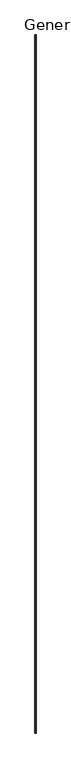
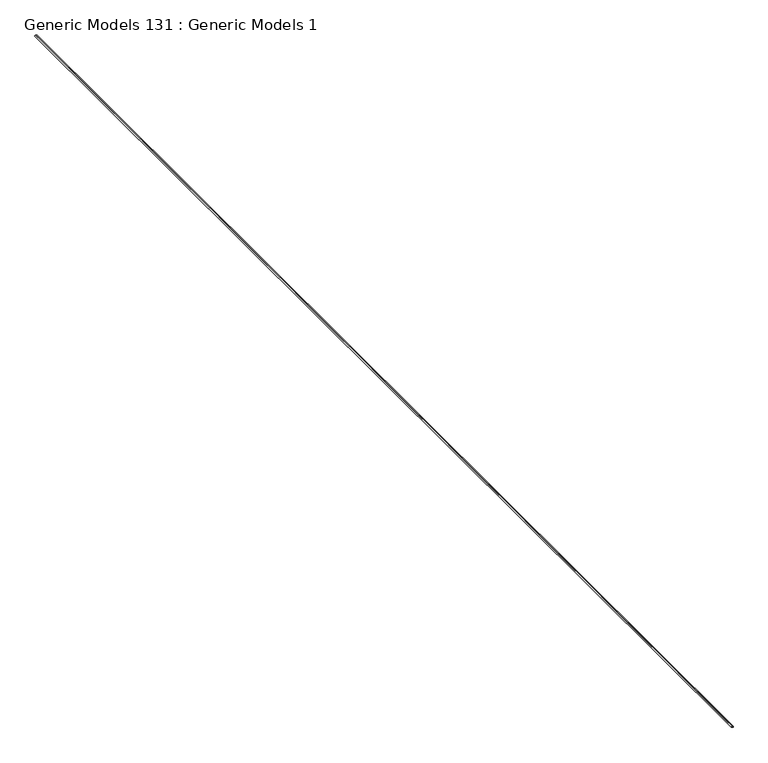
"""IFC4 building model written with IfcOpenShell, lengths in millimetres: proxy geometry, Generic Models 131 : Generic Models 1."""

import ifcopenshell
import ifcopenshell.guid

model = None  # the IFC model being written
_history = None  # IfcOwnerHistory: only IFC2X3 demands one
_inside = {}  # id of a spatial element -> (the spatial element, [elements in it])
_under = {}  # id of a project, library or spatial element -> (it, [spatial elements below it])
_declared = {}  # id of a project -> (the project, [libraries it declares])
_typed = {}  # id of a type object -> (the type object, [elements of that type])
_made_of = {}  # id of a material, layer set ... -> (it, [elements and type objects made of it])


def new_model(schema):
    """Start an empty IFC model of exactly this schema.

    Asked for "IFC4X3", IfcOpenShell would pick the latest addendum, in which some entities
    have other attributes; the version numbers below select the first issue.
    IFC2X3 requires an IfcOwnerHistory on every rooted entity: one is made here for all.
    """
    global model, _history
    if schema == "IFC4X3":
        model = ifcopenshell.file(schema_version=(4, 3, 0, 0))
    else:
        model = ifcopenshell.file(schema=schema)
    _inside.clear()
    _under.clear()
    _declared.clear()
    _typed.clear()
    _made_of.clear()
    _history = None
    if model.schema == "IFC2X3":
        org = make("IfcOrganization", Name="unknown")
        user = make(
            "IfcPersonAndOrganization",
            ThePerson=make("IfcPerson", FamilyName="unknown"),
            TheOrganization=org,
        )
        app = make(
            "IfcApplication",
            ApplicationDeveloper=org,
            Version="unknown",
            ApplicationFullName="unknown",
            ApplicationIdentifier="unknown",
        )
        _history = make(
            "IfcOwnerHistory",
            OwningUser=user,
            OwningApplication=app,
            ChangeAction="ADDED",
            CreationDate=0,
        )
    return model


def make(cls, **values):
    """One entity of the class cls with the attributes given. An attribute that is None is left unset."""
    return model.create_entity(
        cls, **{name: value for name, value in values.items() if value is not None}
    )


def rooted(cls, **values):
    """An entity with a GlobalId (a new one), such as an element, a storey or a relation."""
    return make(cls, GlobalId=ifcopenshell.guid.new(), OwnerHistory=_history, **values)


def si_unit(unit_type, name, prefix=None):
    """IfcSIUnit, for example si_unit("LENGTHUNIT", "METRE", prefix="MILLI")."""
    return make("IfcSIUnit", UnitType=unit_type, Prefix=prefix, Name=name)


def assignment(units):
    """IfcUnitAssignment: the units of a project."""
    return None if units is None else make("IfcUnitAssignment", Units=units)


def point(xyz):
    """IfcCartesianPoint."""
    return None if xyz is None else make("IfcCartesianPoint", Coordinates=xyz)


def direction(xyz):
    """IfcDirection."""
    return None if xyz is None else make("IfcDirection", DirectionRatios=xyz)


def frame(location, z_axis=None, x_axis=None):
    """IfcAxis2Placement3D, a coordinate frame: its origin and axes. An axis left out is left unset."""
    return make(
        "IfcAxis2Placement3D",
        Location=point(location),
        Axis=direction(z_axis),
        RefDirection=direction(x_axis),
    )


def origin():
    """The frame at (0, 0, 0) with its axes left unset."""
    return frame((0.0, 0.0, 0.0))


def place(relative_to, where):
    """IfcLocalPlacement: puts the frame where relative to a parent placement (None: the world)."""
    return make(
        "IfcLocalPlacement", PlacementRelTo=relative_to, RelativePlacement=where
    )


def context(
    kind, dimensions, precision=None, world=None, true_north=None, identifier=None
):
    """IfcGeometricRepresentationContext, for example the 3D "Model" context."""
    return make(
        "IfcGeometricRepresentationContext",
        ContextIdentifier=identifier,
        ContextType=kind,
        CoordinateSpaceDimension=dimensions,
        Precision=precision,
        WorldCoordinateSystem=world,
        TrueNorth=true_north,
    )


def project(units=None, contexts=None):
    """IfcProject with its units and contexts."""
    return rooted(
        "IfcProject",
        Name="project",
        RepresentationContexts=contexts,
        UnitsInContext=assignment(units),
    )


def spatial(cls, under=None, at=None, **own):
    """A site, building, storey or space (cls), placed at a placement, below another one or the project."""
    s = rooted(cls, ObjectPlacement=at, **own)
    if under is not None:
        _under.setdefault(under.id(), (under, []))[1].append(s)
    return s


def polyline(points):
    """IfcPolyline through the points."""
    return make("IfcPolyline", Points=[point(p) for p in points])


def circle_curve(where, radius):
    """IfcCircle in the frame where."""
    return make("IfcCircle", Position=where, Radius=radius)


def ellipse_curve(where, semi_axis1, semi_axis2):
    """IfcEllipse in the frame where."""
    return make(
        "IfcEllipse", Position=where, SemiAxis1=semi_axis1, SemiAxis2=semi_axis2
    )


def trimmed(basis, trim1, trim2, sense, master):
    """IfcTrimmedCurve: the piece of a basis curve between two trims."""
    return make(
        "IfcTrimmedCurve",
        BasisCurve=basis,
        Trim1=trim1,
        Trim2=trim2,
        SenseAgreement=sense,
        MasterRepresentation=master,
    )


def shape(context_of_items, identifier, shape_type, items):
    """IfcShapeRepresentation: the items that make up one representation, for example the "Body"."""
    return make(
        "IfcShapeRepresentation",
        ContextOfItems=context_of_items,
        RepresentationIdentifier=identifier,
        RepresentationType=shape_type,
        Items=items,
    )


def source(mapping_origin, context_of_items, identifier, shape_type, items):
    """IfcRepresentationMap: a shape defined once, which mapped items show again and again."""
    return make(
        "IfcRepresentationMap",
        MappingOrigin=mapping_origin,
        MappedRepresentation=shape(context_of_items, identifier, shape_type, items),
    )


def transform(
    local_origin,
    x_axis=None,
    y_axis=None,
    z_axis=None,
    scale=None,
    scale2=None,
    scale3=None,
    uniform=True,
):
    """IfcCartesianTransformationOperator3D, or its non-uniform kind. x_axis, y_axis, z_axis: its Axis1, 2, 3."""
    if uniform:
        return make(
            "IfcCartesianTransformationOperator3D",
            Axis1=direction(x_axis),
            Axis2=direction(y_axis),
            LocalOrigin=point(local_origin),
            Scale=scale,
            Axis3=direction(z_axis),
        )
    return make(
        "IfcCartesianTransformationOperator3DnonUniform",
        Axis1=direction(x_axis),
        Axis2=direction(y_axis),
        LocalOrigin=point(local_origin),
        Scale=scale,
        Axis3=direction(z_axis),
        Scale2=scale2,
        Scale3=scale3,
    )


def mapped(mapping_source, mapping_target):
    """IfcMappedItem: shows the shape of a source again, moved by a transform."""
    return make(
        "IfcMappedItem", MappingSource=mapping_source, MappingTarget=mapping_target
    )


def made_of(thing, what):
    """Note that an element or type object is made of a material, layer set ...; save() writes the relation."""
    if what is not None:
        _made_of.setdefault(what.id(), (what, []))[1].append(thing)
    return thing


def element(
    cls,
    number,
    at=None,
    inside=None,
    cuts=None,
    type_object=None,
    material=None,
    context=None,
    identifier="Body",
    shape_type=None,
    held_by="IfcProductDefinitionShape",
    body=None,
    shapes=None,
    **own,
):
    """One element of the class cls, such as IfcWall. Its Tag is "e" and its number.

    at: its placement. inside: the storey or other place that contains it. cuts: it is an
    opening in that element (IfcRelVoidsElement). A single representation is given by context,
    identifier, shape_type and body (its items); several are given by shapes. held_by: the class
    of the entity that holds the representations. save() writes the other relations.
    """
    e = rooted(cls, Tag="e%d" % number, ObjectPlacement=at, **own)
    if body is not None:
        shapes = [shape(context, identifier, shape_type, body)]
    if shapes is not None:
        e.Representation = make(held_by, Representations=shapes)
    if inside is not None:
        _inside.setdefault(inside.id(), (inside, []))[1].append(e)
    if cuts is not None:
        rooted(
            "IfcRelVoidsElement", RelatingBuildingElement=cuts, RelatedOpeningElement=e
        )
    if type_object is not None:
        _typed.setdefault(type_object.id(), (type_object, []))[1].append(e)
    return made_of(e, material)


def aggregate(whole, parts):
    """IfcRelAggregates: a whole, such as a stair, and the parts it consists of."""
    return rooted("IfcRelAggregates", RelatingObject=whole, RelatedObjects=parts)


def save(model, path):
    """Write the relations noted so far, then the file.

    IfcRelAggregates (storeys below a building ...), IfcRelContainedInSpatialStructure (elements
    in a storey), IfcRelDefinesByType, IfcRelAssociatesMaterial and IfcRelDeclares: one each for
    every whole, place, type object, material and project.
    """
    for whole, parts in _under.values():
        aggregate(whole, parts)
    for where, things in _inside.values():
        rooted(
            "IfcRelContainedInSpatialStructure",
            RelatedElements=things,
            RelatingStructure=where,
        )
    for kind, things in _typed.values():
        rooted("IfcRelDefinesByType", RelatedObjects=things, RelatingType=kind)
    for what, things in _made_of.values():
        rooted("IfcRelAssociatesMaterial", RelatedObjects=things, RelatingMaterial=what)
    for by, libraries in _declared.values():
        rooted("IfcRelDeclares", RelatingContext=by, RelatedDefinitions=libraries)
    model.write(path)


def plane_surface(at):
    """IfcPlane: the flat surface through the origin of the frame at, square to its z axis."""
    return make("IfcPlane", Position=at)


def cylinder_surface(at, radius):
    """IfcCylindricalSurface: all points at the distance radius from the z axis of the frame at."""
    return make("IfcCylindricalSurface", Position=at, Radius=radius)


def revolved_surface(curve, axis_point, axis_direction):
    """IfcSurfaceOfRevolution: the curve turned about the line through axis_point along axis_direction."""
    return make(
        "IfcSurfaceOfRevolution",
        SweptCurve=make("IfcArbitraryOpenProfileDef", ProfileType="CURVE", Curve=curve),
        AxisPosition=make("IfcAxis1Placement", Location=point(axis_point), Axis=direction(axis_direction)),
    )


def extruded_surface(curve, direction_of_extrusion, depth):
    """IfcSurfaceOfLinearExtrusion: the curve pushed along a direction by depth."""
    return make(
        "IfcSurfaceOfLinearExtrusion",
        SweptCurve=make("IfcArbitraryOpenProfileDef", ProfileType="CURVE", Curve=curve),
        ExtrudedDirection=direction(direction_of_extrusion),
        Depth=depth,
    )


def advanced_brep(points, edges, surfaces, faces):
    """IfcAdvancedBrep: a solid bounded by faces that lie on surfaces and meet in shared edges.

    An edge is (start, end): straight between two places in points (the first is 0);
    or (start, end, curve); or (start, end, curve, False) where it runs against its curve.
    A face is (place in surfaces, loops), or (place, loops, False) where it looks against
    its surface's normal. A loop lists edges by number (the first is 1), with a minus sign
    where the edge is run from its end to its start. The first loop is the outer one.
    """
    corners = [point(p) for p in points]
    vertices = [make("IfcVertexPoint", VertexGeometry=c) for c in corners]
    made = []
    for start, end, *more in edges:
        made.append(
            make(
                "IfcEdgeCurve",
                EdgeStart=vertices[start],
                EdgeEnd=vertices[end],
                EdgeGeometry=more[0] if more else make("IfcPolyline", Points=[corners[start], corners[end]]),
                SameSense=more[1] if len(more) > 1 else True,
            )
        )
    hull = []
    for where, loops, *sense in faces:
        bounds = []
        for j, loop in enumerate(loops):
            ring = [make("IfcOrientedEdge", EdgeElement=made[abs(k) - 1], Orientation=k > 0) for k in loop]
            bounds.append(
                make(
                    "IfcFaceOuterBound" if j == 0 else "IfcFaceBound",
                    Bound=make("IfcEdgeLoop", EdgeList=ring),
                    Orientation=True,
                )
            )
        hull.append(make("IfcAdvancedFace", Bounds=bounds, FaceSurface=surfaces[where], SameSense=sense[0] if sense else True))
    return make("IfcAdvancedBrep", Outer=make("IfcClosedShell", CfsFaces=hull))


def generic_models_131_generic_models_1_40819db8(model_context):
    return source(origin(), model_context, "Body", "AdvancedBrep", [
        advanced_brep(
        [(5019.461606, -1504.2676118, 129170.1348752), (5016.286606, -1504.2676118, 129170.1348752), (5015.3348467, -1504.2676118, 129168.8642166), (5015.3348467, -1504.2676118, 129165.0555337), (5016.286606, -1504.2676118, 129163.7848752), (5019.461606, -1504.2676118, 129163.7848752), (5019.461606, 6382.4323882, 129170.1348752), (5019.461606, 6382.4323882, 129163.7848752), (5016.286606, 6382.4323882, 129163.7848752), (5015.3348467, 6382.4323882, 129165.0555337), (5015.3348467, 6382.4323882, 129168.8642166), (5016.286606, 6382.4323882, 129170.1348752)],
        [
            (0, 1),
            (1, 2, circle_curve(frame((5019.2013465, -1504.2676118, 129166.9598752), z_axis=(0.0, -1.0, 0.0), x_axis=(0.0, 0.0, 1.0)), 4.3100275)),
            (2, 3, ellipse_curve(frame((5011.524106, -1504.2676118, 129166.9598752), z_axis=(0.0, -1.0, 0.0), x_axis=(1.0, 0.0, 0.0)), 4.7625, 3.175)),
            (3, 4, circle_curve(frame((5019.2013465, -1504.2676118, 129166.9598752), z_axis=(0.0, -1.0, 0.0), x_axis=(0.0, 0.0, 1.0)), 4.3100275)),
            (4, 5),
            (5, 0, circle_curve(frame((5022.3763465, -1504.2676118, 129166.9598752), z_axis=(0.0, 1.0, 0.0), x_axis=(0.0, 0.0, 1.0)), 4.3100275)),
            (6, 7, circle_curve(frame((5022.3763465, 6382.4323882, 129166.9598752), z_axis=(0.0, -1.0, 0.0), x_axis=(0.0, 0.0, 1.0)), 4.3100275)),
            (7, 8),
            (8, 9, circle_curve(frame((5019.2013465, 6382.4323882, 129166.9598752), z_axis=(0.0, 1.0, 0.0), x_axis=(0.0, 0.0, 1.0)), 4.3100275)),
            (9, 10, ellipse_curve(frame((5011.524106, 6382.4323882, 129166.9598752), z_axis=(0.0, 1.0, 0.0), x_axis=(1.0, 0.0, 0.0)), 4.7625, 3.175)),
            (10, 11, circle_curve(frame((5019.2013465, 6382.4323882, 129166.9598752), z_axis=(0.0, 1.0, 0.0), x_axis=(0.0, 0.0, 1.0)), 4.3100275)),
            (11, 6),
            (2, 10),
            (9, 3),
            (0, 6),
            (11, 1),
            (8, 4),
            (7, 5),
        ],
        [
            plane_surface(frame((5019.461606, -1504.2676118, 129163.7848752), z_axis=(0.0, -1.0, 0.0), x_axis=(1.0, 0.0, 0.0))),
            plane_surface(frame((5019.461606, 6382.4323882, 129163.7848752), z_axis=(0.0, 1.0, 0.0), x_axis=(1.0, 0.0, 0.0))),
            extruded_surface(trimmed(ellipse_curve(frame((5011.524106, 6382.4323882, 129166.9598752), z_axis=(0.0, -1.0, 0.0), x_axis=(1.0, 0.0, 0.0)), 4.7625, 3.175), [point((5015.3348467, 6382.4323882, 129168.8642166))], [point((5015.3348467, 6382.4323882, 129165.0555337))], True, "CARTESIAN"), (0.0, -7886.7, 0.0), 7886.7),
            plane_surface(frame((5019.461606, -1504.2676118, 129170.1348752), z_axis=(0.0, 0.0, 1.0), x_axis=(0.0, 1.0, 0.0))),
            cylinder_surface(frame((5019.2013465, -1504.2676118, 129166.9598752), z_axis=(0.0, -1.0, 0.0), x_axis=(0.0, 0.0, 1.0)), 4.3100275),
            plane_surface(frame((5016.286606, -1504.2676118, 129163.7848752), z_axis=(0.0, 0.0, -1.0), x_axis=(0.0, 1.0, 0.0))),
            revolved_surface(polyline([(5022.3763465, 6382.4323882, 129171.2699027), (5022.3763465, -1504.2676118, 129171.2699027)]), (5022.3763465, -1504.2676118, 129166.9598752), (0.0, 1.0, 0.0)),
        ],
        [
            (0, [[1, 2, 3, 4, 5, 6]]),
            (1, [[7, 8, 9, 10, 11, 12]]),
            (2, [[-3, 13, -10, 14]]),
            (3, [[-1, 15, -12, 16]]),
            (4, [[-4, -14, -9, 17]]),
            (5, [[-5, -17, -8, 18]]),
            (6, [[-6, -18, -7, -15]]),
            (4, [[-2, -16, -11, -13]]),
        ],
    ),
    ])


if __name__ == "__main__":
    model = new_model("IFC4")
    model_context = context("Model", 3, world=origin())
    ifc_project = project(units=[si_unit("LENGTHUNIT", "METRE", prefix="MILLI")], contexts=[model_context])
    site = spatial("IfcSite", under=ifc_project)
    building = spatial("IfcBuilding", under=site)
    placement = place(None, origin())
    generic_models_131_generic_models_1_shape = generic_models_131_generic_models_1_40819db8(model_context)
    element("IfcBuildingElementProxy", 1, Name="Generic Models 131 : Generic Models 1", ObjectType="Generic Models 131 : Generic Models 1", at=placement, inside=building, context=model_context, shape_type="MappedRepresentation", body=[
        mapped(generic_models_131_generic_models_1_shape, transform((0.0, 0.0, 0.0), x_axis=(1.0, 0.0, 0.0), y_axis=(0.0, 1.0, 0.0), z_axis=(0.0, 0.0, 1.0))),
    ])
    save(model, "model.ifc")

# Revit data of these elements
# Element 1 (IfcBuildingElementProxy, "Generic Models 131 : Generic Models 1")
#   Materials on its faces: "_SEALANT AND BACKROD, IF NEC."
# Materials
#   "_SEALANT AND BACKROD, IF NEC.": class "Generic", colour RGB 190 220 196, transparency 0, Cost = 0
